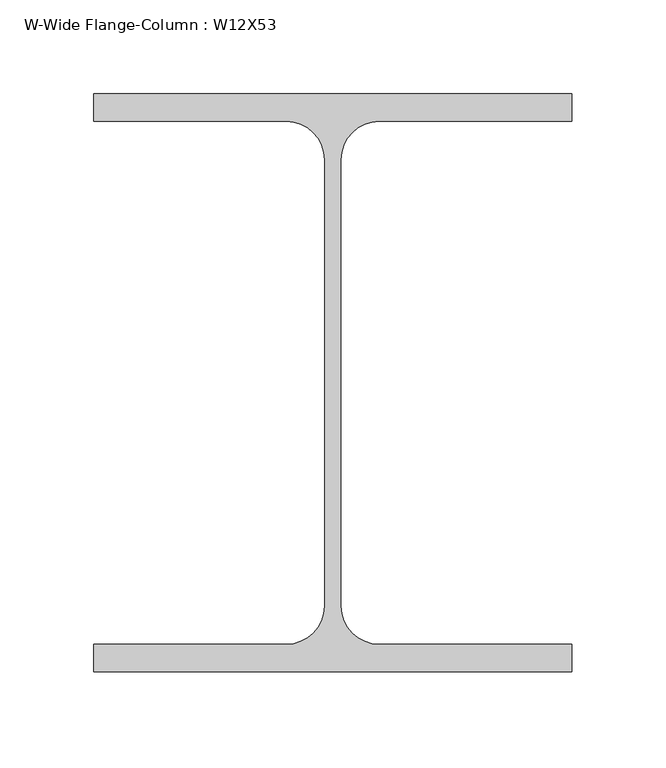
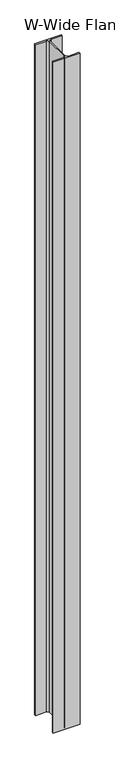
"""IFC4 building model written with IfcOpenShell, lengths in millimetres: column geometry, W-Wide Flange-Column : W12X53."""

from ifc_helpers import new_model, si_unit, point, frame, frame_2d, origin, place, context, project, spatial, polyline, circle_curve, trimmed, segment, composite_curve, outline, extrude, source, transform, mapped, element, save


def w_wide_flange_column_w12x53_4b29bfd7(model_context):
    return source(origin(), model_context, "Body", "SweptSolid", [
        extrude(outline(composite_curve([segment(polyline([(127.0, 153.67), (127.0, 139.065), (24.7015, 139.065)]), True, "CONTINUOUS"), segment(trimmed(circle_curve(frame_2d((24.7015, 118.745)), 20.32), [point((24.7015, 139.065))], [point((4.3815, 118.745))], True, "CARTESIAN"), True, "CONTINUOUS"), segment(polyline([(4.3815, 118.745), (4.3815, -118.745)]), True, "CONTINUOUS"), segment(trimmed(circle_curve(frame_2d((24.7015, -118.745)), 20.32), [point((4.3815, -118.745))], [point((24.7015, -139.065))], True, "CARTESIAN"), True, "CONTINUOUS"), segment(polyline([(24.7015, -139.065), (127.0, -139.065), (127.0, -153.67), (-127.0, -153.67), (-127.0, -139.065), (-24.7015, -139.065)]), True, "CONTINUOUS"), segment(trimmed(circle_curve(frame_2d((-24.7015, -118.745)), 20.32), [point((-24.7015, -139.065))], [point((-4.3815, -118.745))], True, "CARTESIAN"), True, "CONTINUOUS"), segment(polyline([(-4.3815, -118.745), (-4.3815, 118.745)]), True, "CONTINUOUS"), segment(trimmed(circle_curve(frame_2d((-24.7015, 118.745)), 20.32), [point((-4.3815, 118.745))], [point((-24.7015, 139.065))], True, "CARTESIAN"), True, "CONTINUOUS"), segment(polyline([(-24.7015, 139.065), (-127.0, 139.065), (-127.0, 153.67), (127.0, 153.67)]), True, "CONTINUOUS")], self_intersect=False)), frame((0.0, 0.0, 8756.65), z_axis=(0.0, 0.0, 1.0), x_axis=(1.0, 0.0, 0.0)), (0.0, 0.0, 1.0), 6770.3898438),
    ])


if __name__ == "__main__":
    model = new_model("IFC4")
    model_context = context("Model", 3, world=origin())
    ifc_project = project(units=[si_unit("LENGTHUNIT", "METRE", prefix="MILLI")], contexts=[model_context])
    site = spatial("IfcSite", under=ifc_project)
    building = spatial("IfcBuilding", under=site)
    placement = place(None, origin())
    w_wide_flange_column_w12x53_shape = w_wide_flange_column_w12x53_4b29bfd7(model_context)
    element("IfcColumn", 1, ObjectType="W-Wide Flange-Column : W12X53", at=placement, inside=building, context=model_context, shape_type="MappedRepresentation", body=[
        mapped(w_wide_flange_column_w12x53_shape, transform((0.0, 0.0, 0.0), x_axis=(1.0, 0.0, 0.0), y_axis=(0.0, 1.0, 0.0), z_axis=(0.0, 0.0, 1.0))),
    ])
    save(model, "model.ifc")

# Revit data of these elements
# Type "W-Wide Flange-Column : W12X53"
#   Assembly Code = "B10"
#   W = 53
#   bf = 0' - 10"
#   d = 1' - 0.1"
#   k = 0' - 1 3/8"
#   kr = 0' - 0.8"
#   tf = 0' - 0.575"
#   tw = 0' - 0.345"
#   A = 0.108333 SF
#   Structural Material [instance default] = Steel ASTM A992
# Element 1 (IfcColumn, "W-Wide Flange-Column : W12X53")
#   Materials on its faces: "Steel ASTM A992"
# Materials
#   "Steel ASTM A992": class "Metal", colour RGB 199 199 199, transparency 0, Description = "Structural steel 50ksi", Cost = 0
